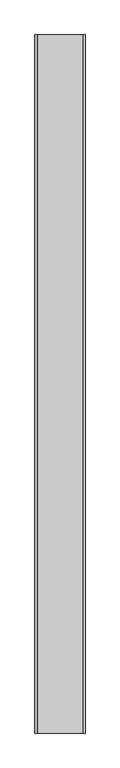
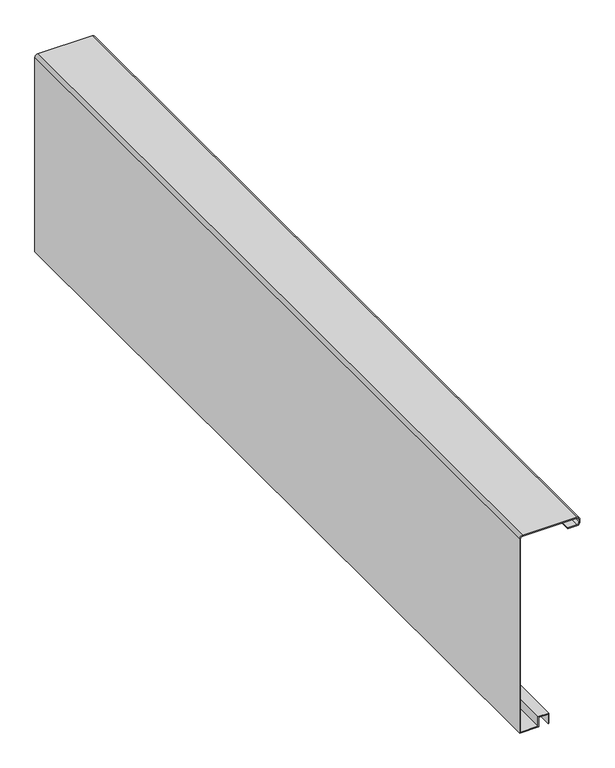
"""IFC4 building model written with IfcOpenShell, lengths in millimetres: proxy geometry, Flashing7:Flashing008:290665 : Flashing7:Flashing008:290665."""

from ifc_helpers import new_model, si_unit, point, frame, frame_2d, origin, place, context, project, spatial, polyline, circle_curve, trimmed, segment, composite_curve, outline, extrude, source, transform, mapped, element, save


def generic_models_b361f573(model_context):
    return source(origin(), model_context, "Body", "SweptSolid", [
        extrude(outline(composite_curve([segment(polyline([(43032.1617235, -1721.8458725), (43518.4785937, -1721.8458725)]), True, "CONTINUOUS"), segment(trimmed(circle_curve(frame_2d((43518.4785937, -1716.7658725)), 5.08), [point((43518.4785937, -1721.8458725))], [point((43523.5585937, -1716.7658725))], True, "CARTESIAN"), True, "CONTINUOUS"), segment(polyline([(43523.5585937, -1716.7658725), (43523.5585937, -1587.4258725)]), True, "CONTINUOUS"), segment(trimmed(circle_curve(frame_2d((43518.4785937, -1587.4258725)), 5.08), [point((43523.5585937, -1587.4258725))], [point((43518.4785937, -1582.3458725))], True, "CARTESIAN"), True, "CONTINUOUS"), segment(polyline([(43518.4785937, -1582.3458725), (43512.0721875, -1582.3458725)]), True, "CONTINUOUS"), segment(trimmed(circle_curve(frame_2d((43512.0721875, -1587.4258725)), 5.08), [point((43512.0721875, -1582.3458725))], [point((43506.9921875, -1587.4258725))], True, "CARTESIAN"), True, "CONTINUOUS"), segment(polyline([(43506.9921875, -1587.4258725), (43506.9921875, -1608.7223373), (43504.9921875, -1608.7223373), (43504.9921875, -1587.4258725)]), True, "CONTINUOUS"), segment(trimmed(circle_curve(frame_2d((43512.0721875, -1587.4258725)), 7.08), [point((43504.9921875, -1587.4258725))], [point((43512.0721875, -1580.3458725))], False, "CARTESIAN"), True, "CONTINUOUS"), segment(polyline([(43512.0721875, -1580.3458725), (43518.4785937, -1580.3458725)]), True, "CONTINUOUS"), segment(trimmed(circle_curve(frame_2d((43518.4785937, -1587.4258725)), 7.08), [point((43518.4785937, -1580.3458725))], [point((43525.5585937, -1587.4258725))], False, "CARTESIAN"), True, "CONTINUOUS"), segment(polyline([(43525.5585937, -1587.4258725), (43525.5585937, -1716.7658725)]), True, "CONTINUOUS"), segment(trimmed(circle_curve(frame_2d((43518.4785937, -1716.7658725)), 7.08), [point((43525.5585937, -1716.7658725))], [point((43518.4785937, -1723.8458725))], False, "CARTESIAN"), True, "CONTINUOUS"), segment(polyline([(43518.4785937, -1723.8458725), (43030.1617235, -1723.8458725), (43030.1617235, -1678.5207187), (43054.2082994, -1678.5207187), (43054.2082994, -1656.1205016), (43030.1617235, -1656.1205016), (43030.1617235, -1654.1205016), (43056.2082994, -1654.1205016), (43056.2082994, -1680.5207187), (43032.1617235, -1680.5207187), (43032.1617235, -1721.8458725)]), True, "CONTINUOUS")], self_intersect=False)), frame((0.0, 8260.4857132, 0.0), z_axis=(0.0, 1.0, 0.0), x_axis=(0.0, 0.0, 1.0)), (0.0, 0.0, 1.0), 2000.0),
    ])


if __name__ == "__main__":
    model = new_model("IFC4")
    model_context = context("Model", 3, world=origin())
    ifc_project = project(units=[si_unit("LENGTHUNIT", "METRE", prefix="MILLI")], contexts=[model_context])
    site = spatial("IfcSite", under=ifc_project)
    building = spatial("IfcBuilding", under=site)
    placement = place(None, origin())
    generic_models_shape = generic_models_b361f573(model_context)
    element("IfcBuildingElementProxy", 1, Name="Flashing7:Flashing008:290665 : Flashing7:Flashing008:290665", ObjectType="Flashing7:Flashing008:290665 : Flashing7:Flashing008:290665", at=placement, inside=building, context=model_context, shape_type="MappedRepresentation", body=[
        mapped(generic_models_shape, transform((0.0, 0.0, 0.0), x_axis=(1.0, 0.0, 0.0), y_axis=(0.0, 1.0, 0.0), z_axis=(0.0, 0.0, 1.0))),
    ])
    save(model, "model.ifc")

# Revit data of these elements
# Type "Flashing7:Flashing008:290665 : Flashing7:Flashing008:290665"
#   NameOverride = "Flashing7:Flashing008:290665"
#   ObjectTypeOverride = "Flashing7:Flashing008"
#   Reference = "Flashing008"
#   Category = "Generic Models"
#   Tag = "290665"
# Element 1 (IfcBuildingElementProxy, "Flashing7:Flashing008:290665 : Flashing7:Flashing008:290665")
#   Materials on its faces: "BRAKE METAL EAVE TRIM TO MATCH STANDING SEAM COLOR"
# Materials
#   "BRAKE METAL EAVE TRIM TO MATCH STANDING SEAM COLOR": class "Unassigned", colour RGB 128 128 128, transparency 0, Cost = 0
